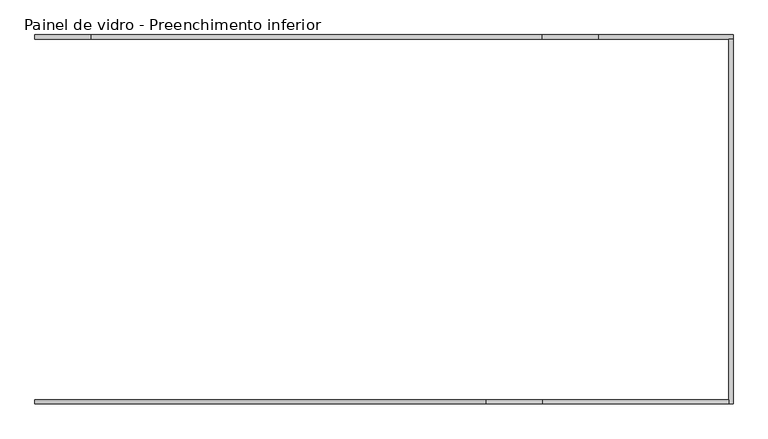
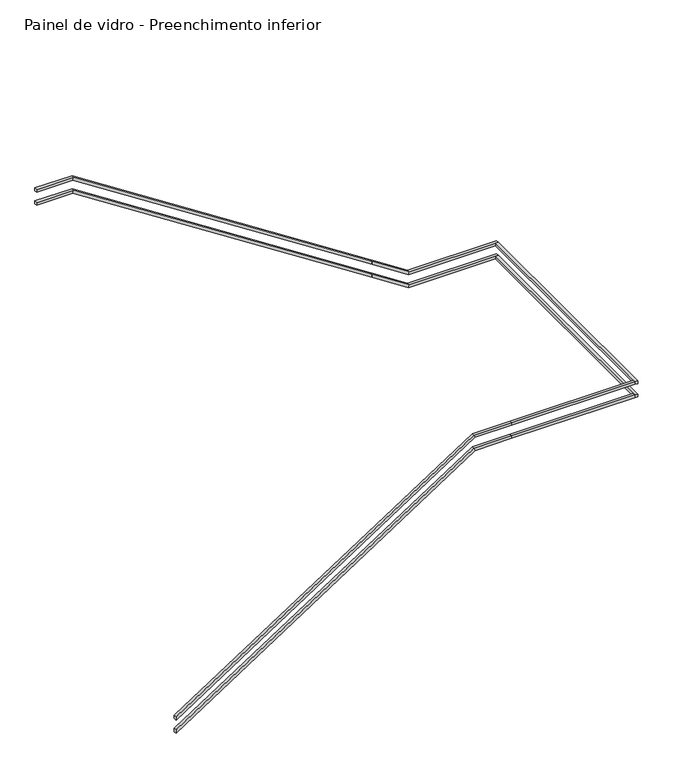
"""IFC4 building model written with IfcOpenShell, lengths in millimetres: railing geometry, Painel de vidro - Preenchimento inferior."""

from ifc_helpers import new_model, si_unit, origin, place, context, project, spatial, faceted_brep, source, transform, mapped, element, save


def painel_de_vidro_preenchimento_inferior_ea4134fb(model_context):
    return source(origin(), model_context, "Body", "Brep", [
        faceted_brep([(5899.9999996, 3563.4, 1275.0), (5899.9999996, 3583.4, 1275.0), (5899.9999996, 3583.4, 1251.1664436), (5899.9999996, 3563.4, 1251.1664436), (8059.9999996, 3563.4, 2675.0), (8059.9999996, 3583.4, 2675.0), (8065.9146294, 3583.4, 2655.0), (8065.9146294, 3563.4, 2655.0), (8329.9999996, 3563.4, 2675.0), (8329.9999996, 3563.4, 2655.0), (8329.9999996, 3583.4, 2655.0), (8329.9999996, 3583.4, 2675.0)], [[[0, 1, 2, 3]], [[1, 0, 4, 5]], [[2, 1, 5, 6]], [[3, 2, 6, 7]], [[0, 3, 7, 4]], [[8, 9, 10, 11]], [[5, 4, 8, 11]], [[6, 5, 11, 10]], [[7, 6, 10, 9]], [[4, 7, 9, 8]]]),
        faceted_brep([(8329.9999996, 3563.4, 2675.0), (8329.9999996, 3583.4, 2675.0), (8329.9999996, 3583.4, 2655.0), (8329.9999996, 3563.4, 2655.0), (9224.5999996, 3563.4, 2675.0), (9224.5999996, 3563.4, 2655.0), (9224.5999996, 3583.4, 2655.0), (9224.5999996, 3583.4, 2675.0)], [[[0, 1, 2, 3]], [[4, 5, 6, 7]], [[1, 0, 4, 7]], [[2, 1, 7, 6]], [[3, 2, 6, 5]], [[0, 3, 5, 4]]]),
        faceted_brep([(9244.5999996, 3563.4, 2675.0), (9224.5999996, 3563.4, 2675.0), (9224.5999996, 3563.4, 2655.0), (9244.5999996, 3563.4, 2655.0), (9244.5999996, 5312.6, 2675.0), (9244.5999996, 5312.6, 2655.0), (9224.5999996, 5312.6, 2655.0), (9224.5999996, 5312.6, 2675.0)], [[[0, 1, 2, 3]], [[4, 5, 6, 7]], [[1, 0, 4, 7]], [[2, 1, 7, 6]], [[3, 2, 6, 5]], [[0, 3, 5, 4]]]),
        faceted_brep([(9244.5999996, 5332.6, 2675.0), (9244.5999996, 5312.6, 2675.0), (9244.5999996, 5312.6, 2655.0), (9244.5999996, 5332.6, 2655.0), (8599.9999996, 5332.6, 2675.0), (8599.9999996, 5312.6, 2675.0), (8594.0853698, 5312.6, 2655.0), (8594.0853698, 5332.6, 2655.0), (8329.9999996, 5332.6, 2850.0), (8329.9999996, 5332.6, 2826.1664436), (8329.9999996, 5312.6, 2826.1664436), (8329.9999996, 5312.6, 2850.0)], [[[0, 1, 2, 3]], [[1, 0, 4, 5]], [[2, 1, 5, 6]], [[3, 2, 6, 7]], [[0, 3, 7, 4]], [[8, 9, 10, 11]], [[5, 4, 8, 11]], [[6, 5, 11, 10]], [[7, 6, 10, 9]], [[4, 7, 9, 8]]]),
        faceted_brep([(8329.9999996, 5332.6, 2850.0), (8329.9999996, 5312.6, 2850.0), (8329.9999996, 5312.6, 2826.1664436), (8329.9999996, 5332.6, 2826.1664436), (6169.9999996, 5332.6, 4250.0), (6169.9999996, 5312.6, 4250.0), (6164.0853698, 5312.6, 4230.0), (6164.0853698, 5332.6, 4230.0), (5899.9999996, 5332.6, 4250.0), (5899.9999996, 5332.6, 4230.0), (5899.9999996, 5312.6, 4230.0), (5899.9999996, 5312.6, 4250.0)], [[[0, 1, 2, 3]], [[1, 0, 4, 5]], [[2, 1, 5, 6]], [[3, 2, 6, 7]], [[0, 3, 7, 4]], [[8, 9, 10, 11]], [[5, 4, 8, 11]], [[6, 5, 11, 10]], [[7, 6, 10, 9]], [[4, 7, 9, 8]]]),
        faceted_brep([(5899.9999996, 3563.4, 1175.0), (5899.9999996, 3583.4, 1175.0), (5899.9999996, 3583.4, 1151.1664436), (5899.9999996, 3563.4, 1151.1664436), (8059.9999996, 3563.4, 2575.0), (8059.9999996, 3583.4, 2575.0), (8065.9146294, 3583.4, 2555.0), (8065.9146294, 3563.4, 2555.0), (8329.9999996, 3563.4, 2575.0), (8329.9999996, 3563.4, 2555.0), (8329.9999996, 3583.4, 2555.0), (8329.9999996, 3583.4, 2575.0)], [[[0, 1, 2, 3]], [[1, 0, 4, 5]], [[2, 1, 5, 6]], [[3, 2, 6, 7]], [[0, 3, 7, 4]], [[8, 9, 10, 11]], [[5, 4, 8, 11]], [[6, 5, 11, 10]], [[7, 6, 10, 9]], [[4, 7, 9, 8]]]),
        faceted_brep([(8329.9999996, 3563.4, 2575.0), (8329.9999996, 3583.4, 2575.0), (8329.9999996, 3583.4, 2555.0), (8329.9999996, 3563.4, 2555.0), (9224.5999996, 3563.4, 2575.0), (9224.5999996, 3563.4, 2555.0), (9224.5999996, 3583.4, 2555.0), (9224.5999996, 3583.4, 2575.0)], [[[0, 1, 2, 3]], [[4, 5, 6, 7]], [[1, 0, 4, 7]], [[2, 1, 7, 6]], [[3, 2, 6, 5]], [[0, 3, 5, 4]]]),
        faceted_brep([(9244.5999996, 3563.4, 2575.0), (9224.5999996, 3563.4, 2575.0), (9224.5999996, 3563.4, 2555.0), (9244.5999996, 3563.4, 2555.0), (9244.5999996, 5312.6, 2575.0), (9244.5999996, 5312.6, 2555.0), (9224.5999996, 5312.6, 2555.0), (9224.5999996, 5312.6, 2575.0)], [[[0, 1, 2, 3]], [[4, 5, 6, 7]], [[1, 0, 4, 7]], [[2, 1, 7, 6]], [[3, 2, 6, 5]], [[0, 3, 5, 4]]]),
        faceted_brep([(9244.5999996, 5332.6, 2575.0), (9244.5999996, 5312.6, 2575.0), (9244.5999996, 5312.6, 2555.0), (9244.5999996, 5332.6, 2555.0), (8599.9999996, 5332.6, 2575.0), (8599.9999996, 5312.6, 2575.0), (8594.0853698, 5312.6, 2555.0), (8594.0853698, 5332.6, 2555.0), (8329.9999996, 5332.6, 2750.0), (8329.9999996, 5332.6, 2726.1664436), (8329.9999996, 5312.6, 2726.1664436), (8329.9999996, 5312.6, 2750.0)], [[[0, 1, 2, 3]], [[1, 0, 4, 5]], [[2, 1, 5, 6]], [[3, 2, 6, 7]], [[0, 3, 7, 4]], [[8, 9, 10, 11]], [[5, 4, 8, 11]], [[6, 5, 11, 10]], [[7, 6, 10, 9]], [[4, 7, 9, 8]]]),
        faceted_brep([(8329.9999996, 5332.6, 2750.0), (8329.9999996, 5312.6, 2750.0), (8329.9999996, 5312.6, 2726.1664436), (8329.9999996, 5332.6, 2726.1664436), (6169.9999996, 5332.6, 4150.0), (6169.9999996, 5312.6, 4150.0), (6164.0853698, 5312.6, 4130.0), (6164.0853698, 5332.6, 4130.0), (5899.9999996, 5332.6, 4150.0), (5899.9999996, 5332.6, 4130.0), (5899.9999996, 5312.6, 4130.0), (5899.9999996, 5312.6, 4150.0)], [[[0, 1, 2, 3]], [[1, 0, 4, 5]], [[2, 1, 5, 6]], [[3, 2, 6, 7]], [[0, 3, 7, 4]], [[8, 9, 10, 11]], [[5, 4, 8, 11]], [[6, 5, 11, 10]], [[7, 6, 10, 9]], [[4, 7, 9, 8]]]),
    ])


if __name__ == "__main__":
    model = new_model("IFC4")
    model_context = context("Model", 3, world=origin())
    ifc_project = project(units=[si_unit("LENGTHUNIT", "METRE", prefix="MILLI")], contexts=[model_context])
    site = spatial("IfcSite", under=ifc_project)
    building = spatial("IfcBuilding", under=site)
    placement = place(None, origin())
    painel_de_vidro_preenchimento_inferior_shape = painel_de_vidro_preenchimento_inferior_ea4134fb(model_context)
    element("IfcRailing", 1, ObjectType="Painel de vidro - Preenchimento inferior", at=placement, inside=building, context=model_context, shape_type="MappedRepresentation", body=[
        mapped(painel_de_vidro_preenchimento_inferior_shape, transform((0.0, 0.0, 0.0), x_axis=(1.0, 0.0, 0.0), y_axis=(0.0, 1.0, 0.0), z_axis=(0.0, 0.0, 1.0))),
    ])
    save(model, "model.ifc")
